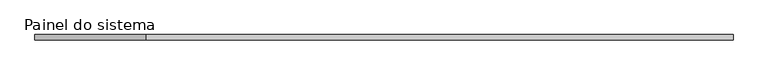
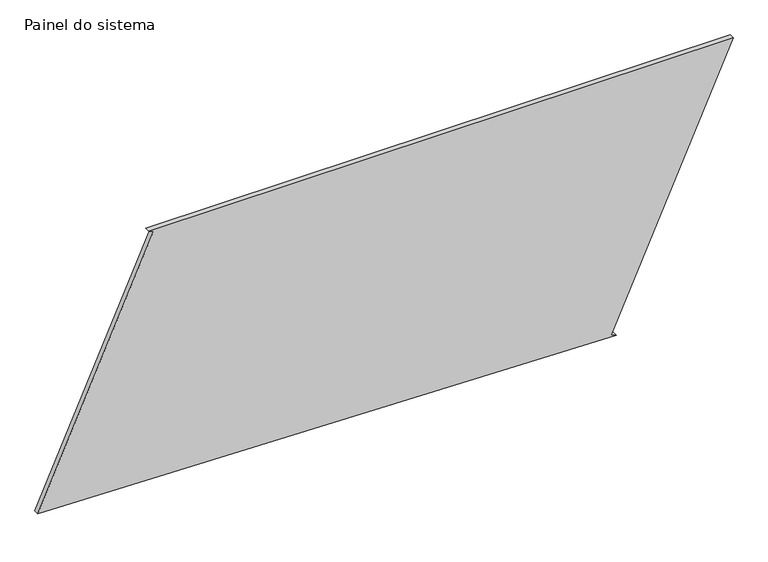
"""IFC4 building model written with IfcOpenShell, lengths in millimetres: plate geometry, Painel do sistema : Envidraçado."""

from ifc_helpers import new_model, si_unit, frame, origin, place, context, project, spatial, polyline, outline, extrude, source, transform, mapped, element, save


def painel_do_sistema_c8b3eec3(model_context):
    return source(origin(), model_context, "Body", "SweptSolid", [
        extrude(outline(polyline([(0.0, 1101.7047789), (10.2299965, 1078.8936595), (1306.5841728, 1660.2635817), (1306.5841728, -1131.8275116), (1296.3541762, -1109.0163921), (67.1684736, -1660.2635817), (0.0, 1101.7047789)])), frame((0.0, 24.5, 0.0), z_axis=(0.0, 1.0, 0.0), x_axis=(0.0, 0.0, 1.0)), (0.0, 0.0, 1.0), 25.0),
    ])


if __name__ == "__main__":
    model = new_model("IFC4")
    model_context = context("Model", 3, world=origin())
    ifc_project = project(units=[si_unit("LENGTHUNIT", "METRE", prefix="MILLI")], contexts=[model_context])
    site = spatial("IfcSite", under=ifc_project)
    building = spatial("IfcBuilding", under=site)
    placement = place(None, origin())
    painel_do_sistema_shape = painel_do_sistema_c8b3eec3(model_context)
    element("IfcPlate", 1, ObjectType="Painel do sistema : Envidraçado", at=placement, inside=building, context=model_context, shape_type="MappedRepresentation", body=[
        mapped(painel_do_sistema_shape, transform((0.0, 0.0, 0.0), x_axis=(1.0, 0.0, 0.0), y_axis=(0.0, 1.0, 0.0), z_axis=(0.0, 0.0, 1.0))),
    ])
    save(model, "model.ifc")

# Revit data of these elements
# Type "Painel do sistema : Envidraçado"
#   Construction Type Id = "GSP4R"
#   Analytic Construction = "Vidraça única Pilkington 1/8 pol"
#   Visual Light Transmittance = 0.9
#   Solar Heat Gain Coefficient = 0.86
#   Heat Transfer Coefficient (U) = 6.7069 W/(m²·K)
# Element 1 (IfcPlate, "Painel do sistema : Envidraçado")
#   Materials on its faces: "Vidro"
# Materials
#   "Vidro": class "Vidro", colour RGB 0 128 192, transparency 0.9, Description = "Vidro de sílica", Cost = 0
